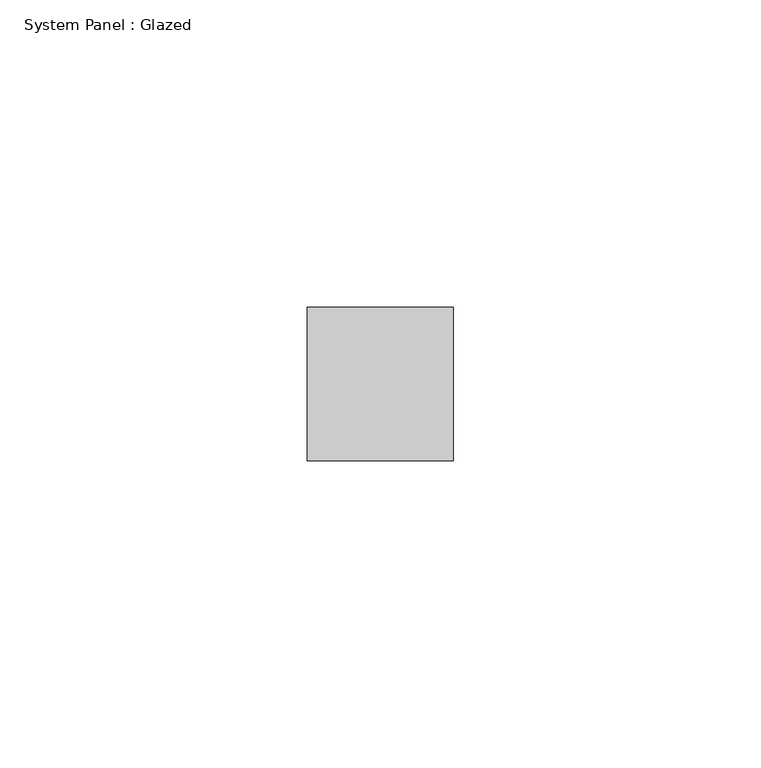
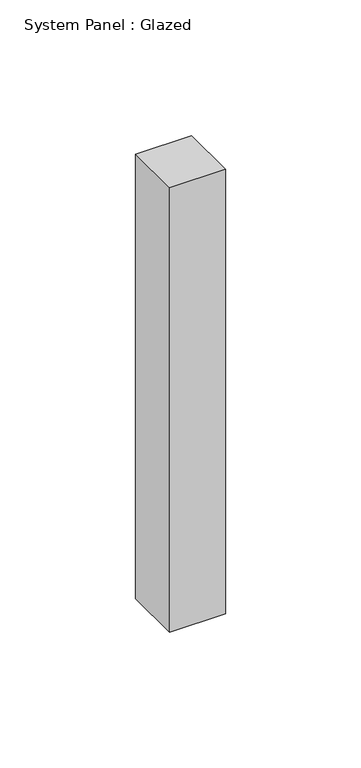
"""IFC4 building model written with IfcOpenShell, lengths in millimetres: plate geometry, System Panel : Glazed."""

from ifc_helpers import new_model, si_unit, origin, origin_with_axes, place, context, project, spatial, polyline, outline, extrude, source, transform, mapped, element, save


def system_panel_glazed_aeb916ba(model_context):
    return source(origin(), model_context, "Body", "SweptSolid", [
        extrude(outline(polyline([(11.9133707, 24.5), (-11.9133707, 24.5), (-11.9133707, 49.5), (11.9133707, 49.5), (11.9133707, 24.5)])), origin_with_axes(), (0.0, 0.0, 1.0), 200.0),
    ])


if __name__ == "__main__":
    model = new_model("IFC4")
    model_context = context("Model", 3, world=origin())
    ifc_project = project(units=[si_unit("LENGTHUNIT", "METRE", prefix="MILLI")], contexts=[model_context])
    site = spatial("IfcSite", under=ifc_project)
    building = spatial("IfcBuilding", under=site)
    placement = place(None, origin())
    system_panel_glazed_shape = system_panel_glazed_aeb916ba(model_context)
    element("IfcPlate", 1, ObjectType="System Panel : Glazed", at=placement, inside=building, context=model_context, shape_type="MappedRepresentation", body=[
        mapped(system_panel_glazed_shape, transform((0.0, 0.0, 0.0), x_axis=(1.0, 0.0, 0.0), y_axis=(0.0, 1.0, 0.0), z_axis=(0.0, 0.0, 1.0))),
    ])
    save(model, "model.ifc")

# Revit data of these elements
# Element 1 (IfcPlate, "System Panel : Glazed")
#   Materials on its faces: "Glass"
# Materials
#   "Glass": class "Glass", colour RGB 218 227 224, transparency 0.85, Description = "Soda Lime Glass", Cost = 0
